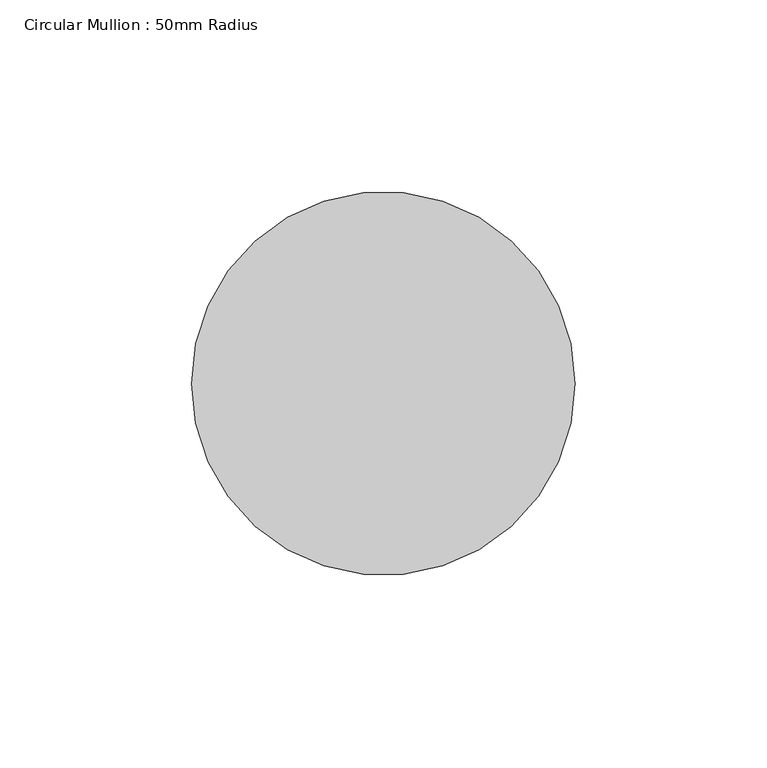
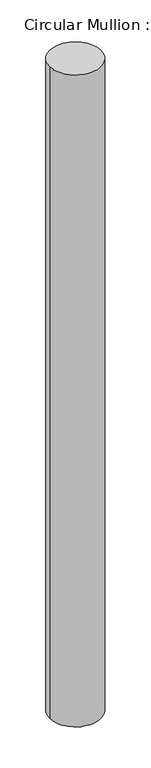
"""IFC4 building model written with IfcOpenShell, lengths in millimetres: member geometry, Circular Mullion : 50mm Radius."""

import ifcopenshell
import ifcopenshell.guid

model = None  # the IFC model being written
_history = None  # IfcOwnerHistory: only IFC2X3 demands one
_inside = {}  # id of a spatial element -> (the spatial element, [elements in it])
_under = {}  # id of a project, library or spatial element -> (it, [spatial elements below it])
_declared = {}  # id of a project -> (the project, [libraries it declares])
_typed = {}  # id of a type object -> (the type object, [elements of that type])
_made_of = {}  # id of a material, layer set ... -> (it, [elements and type objects made of it])


def new_model(schema):
    """Start an empty IFC model of exactly this schema.

    Asked for "IFC4X3", IfcOpenShell would pick the latest addendum, in which some entities
    have other attributes; the version numbers below select the first issue.
    IFC2X3 requires an IfcOwnerHistory on every rooted entity: one is made here for all.
    """
    global model, _history
    if schema == "IFC4X3":
        model = ifcopenshell.file(schema_version=(4, 3, 0, 0))
    else:
        model = ifcopenshell.file(schema=schema)
    _inside.clear()
    _under.clear()
    _declared.clear()
    _typed.clear()
    _made_of.clear()
    _history = None
    if model.schema == "IFC2X3":
        org = make("IfcOrganization", Name="unknown")
        user = make(
            "IfcPersonAndOrganization",
            ThePerson=make("IfcPerson", FamilyName="unknown"),
            TheOrganization=org,
        )
        app = make(
            "IfcApplication",
            ApplicationDeveloper=org,
            Version="unknown",
            ApplicationFullName="unknown",
            ApplicationIdentifier="unknown",
        )
        _history = make(
            "IfcOwnerHistory",
            OwningUser=user,
            OwningApplication=app,
            ChangeAction="ADDED",
            CreationDate=0,
        )
    return model


def make(cls, **values):
    """One entity of the class cls with the attributes given. An attribute that is None is left unset."""
    return model.create_entity(
        cls, **{name: value for name, value in values.items() if value is not None}
    )


def rooted(cls, **values):
    """An entity with a GlobalId (a new one), such as an element, a storey or a relation."""
    return make(cls, GlobalId=ifcopenshell.guid.new(), OwnerHistory=_history, **values)


def si_unit(unit_type, name, prefix=None):
    """IfcSIUnit, for example si_unit("LENGTHUNIT", "METRE", prefix="MILLI")."""
    return make("IfcSIUnit", UnitType=unit_type, Prefix=prefix, Name=name)


def assignment(units):
    """IfcUnitAssignment: the units of a project."""
    return None if units is None else make("IfcUnitAssignment", Units=units)


def point(xyz):
    """IfcCartesianPoint."""
    return None if xyz is None else make("IfcCartesianPoint", Coordinates=xyz)


def direction(xyz):
    """IfcDirection."""
    return None if xyz is None else make("IfcDirection", DirectionRatios=xyz)


def frame(location, z_axis=None, x_axis=None):
    """IfcAxis2Placement3D, a coordinate frame: its origin and axes. An axis left out is left unset."""
    return make(
        "IfcAxis2Placement3D",
        Location=point(location),
        Axis=direction(z_axis),
        RefDirection=direction(x_axis),
    )


def origin():
    """The frame at (0, 0, 0) with its axes left unset."""
    return frame((0.0, 0.0, 0.0))


def place(relative_to, where):
    """IfcLocalPlacement: puts the frame where relative to a parent placement (None: the world)."""
    return make(
        "IfcLocalPlacement", PlacementRelTo=relative_to, RelativePlacement=where
    )


def context(
    kind, dimensions, precision=None, world=None, true_north=None, identifier=None
):
    """IfcGeometricRepresentationContext, for example the 3D "Model" context."""
    return make(
        "IfcGeometricRepresentationContext",
        ContextIdentifier=identifier,
        ContextType=kind,
        CoordinateSpaceDimension=dimensions,
        Precision=precision,
        WorldCoordinateSystem=world,
        TrueNorth=true_north,
    )


def project(units=None, contexts=None):
    """IfcProject with its units and contexts."""
    return rooted(
        "IfcProject",
        Name="project",
        RepresentationContexts=contexts,
        UnitsInContext=assignment(units),
    )


def spatial(cls, under=None, at=None, **own):
    """A site, building, storey or space (cls), placed at a placement, below another one or the project."""
    s = rooted(cls, ObjectPlacement=at, **own)
    if under is not None:
        _under.setdefault(under.id(), (under, []))[1].append(s)
    return s


def ellipse_curve(where, semi_axis1, semi_axis2):
    """IfcEllipse in the frame where."""
    return make(
        "IfcEllipse", Position=where, SemiAxis1=semi_axis1, SemiAxis2=semi_axis2
    )


def shape(context_of_items, identifier, shape_type, items):
    """IfcShapeRepresentation: the items that make up one representation, for example the "Body"."""
    return make(
        "IfcShapeRepresentation",
        ContextOfItems=context_of_items,
        RepresentationIdentifier=identifier,
        RepresentationType=shape_type,
        Items=items,
    )


def source(mapping_origin, context_of_items, identifier, shape_type, items):
    """IfcRepresentationMap: a shape defined once, which mapped items show again and again."""
    return make(
        "IfcRepresentationMap",
        MappingOrigin=mapping_origin,
        MappedRepresentation=shape(context_of_items, identifier, shape_type, items),
    )


def transform(
    local_origin,
    x_axis=None,
    y_axis=None,
    z_axis=None,
    scale=None,
    scale2=None,
    scale3=None,
    uniform=True,
):
    """IfcCartesianTransformationOperator3D, or its non-uniform kind. x_axis, y_axis, z_axis: its Axis1, 2, 3."""
    if uniform:
        return make(
            "IfcCartesianTransformationOperator3D",
            Axis1=direction(x_axis),
            Axis2=direction(y_axis),
            LocalOrigin=point(local_origin),
            Scale=scale,
            Axis3=direction(z_axis),
        )
    return make(
        "IfcCartesianTransformationOperator3DnonUniform",
        Axis1=direction(x_axis),
        Axis2=direction(y_axis),
        LocalOrigin=point(local_origin),
        Scale=scale,
        Axis3=direction(z_axis),
        Scale2=scale2,
        Scale3=scale3,
    )


def mapped(mapping_source, mapping_target):
    """IfcMappedItem: shows the shape of a source again, moved by a transform."""
    return make(
        "IfcMappedItem", MappingSource=mapping_source, MappingTarget=mapping_target
    )


def made_of(thing, what):
    """Note that an element or type object is made of a material, layer set ...; save() writes the relation."""
    if what is not None:
        _made_of.setdefault(what.id(), (what, []))[1].append(thing)
    return thing


def element(
    cls,
    number,
    at=None,
    inside=None,
    cuts=None,
    type_object=None,
    material=None,
    context=None,
    identifier="Body",
    shape_type=None,
    held_by="IfcProductDefinitionShape",
    body=None,
    shapes=None,
    **own,
):
    """One element of the class cls, such as IfcWall. Its Tag is "e" and its number.

    at: its placement. inside: the storey or other place that contains it. cuts: it is an
    opening in that element (IfcRelVoidsElement). A single representation is given by context,
    identifier, shape_type and body (its items); several are given by shapes. held_by: the class
    of the entity that holds the representations. save() writes the other relations.
    """
    e = rooted(cls, Tag="e%d" % number, ObjectPlacement=at, **own)
    if body is not None:
        shapes = [shape(context, identifier, shape_type, body)]
    if shapes is not None:
        e.Representation = make(held_by, Representations=shapes)
    if inside is not None:
        _inside.setdefault(inside.id(), (inside, []))[1].append(e)
    if cuts is not None:
        rooted(
            "IfcRelVoidsElement", RelatingBuildingElement=cuts, RelatedOpeningElement=e
        )
    if type_object is not None:
        _typed.setdefault(type_object.id(), (type_object, []))[1].append(e)
    return made_of(e, material)


def aggregate(whole, parts):
    """IfcRelAggregates: a whole, such as a stair, and the parts it consists of."""
    return rooted("IfcRelAggregates", RelatingObject=whole, RelatedObjects=parts)


def save(model, path):
    """Write the relations noted so far, then the file.

    IfcRelAggregates (storeys below a building ...), IfcRelContainedInSpatialStructure (elements
    in a storey), IfcRelDefinesByType, IfcRelAssociatesMaterial and IfcRelDeclares: one each for
    every whole, place, type object, material and project.
    """
    for whole, parts in _under.values():
        aggregate(whole, parts)
    for where, things in _inside.values():
        rooted(
            "IfcRelContainedInSpatialStructure",
            RelatedElements=things,
            RelatingStructure=where,
        )
    for kind, things in _typed.values():
        rooted("IfcRelDefinesByType", RelatedObjects=things, RelatingType=kind)
    for what, things in _made_of.values():
        rooted("IfcRelAssociatesMaterial", RelatedObjects=things, RelatingMaterial=what)
    for by, libraries in _declared.values():
        rooted("IfcRelDeclares", RelatingContext=by, RelatedDefinitions=libraries)
    model.write(path)


def plane_surface(at):
    """IfcPlane: the flat surface through the origin of the frame at, square to its z axis."""
    return make("IfcPlane", Position=at)


def cylinder_surface(at, radius):
    """IfcCylindricalSurface: all points at the distance radius from the z axis of the frame at."""
    return make("IfcCylindricalSurface", Position=at, Radius=radius)


def advanced_brep(points, edges, surfaces, faces):
    """IfcAdvancedBrep: a solid bounded by faces that lie on surfaces and meet in shared edges.

    An edge is (start, end): straight between two places in points (the first is 0);
    or (start, end, curve); or (start, end, curve, False) where it runs against its curve.
    A face is (place in surfaces, loops), or (place, loops, False) where it looks against
    its surface's normal. A loop lists edges by number (the first is 1), with a minus sign
    where the edge is run from its end to its start. The first loop is the outer one.
    """
    corners = [point(p) for p in points]
    vertices = [make("IfcVertexPoint", VertexGeometry=c) for c in corners]
    made = []
    for start, end, *more in edges:
        made.append(
            make(
                "IfcEdgeCurve",
                EdgeStart=vertices[start],
                EdgeEnd=vertices[end],
                EdgeGeometry=more[0] if more else make("IfcPolyline", Points=[corners[start], corners[end]]),
                SameSense=more[1] if len(more) > 1 else True,
            )
        )
    hull = []
    for where, loops, *sense in faces:
        bounds = []
        for j, loop in enumerate(loops):
            ring = [make("IfcOrientedEdge", EdgeElement=made[abs(k) - 1], Orientation=k > 0) for k in loop]
            bounds.append(
                make(
                    "IfcFaceOuterBound" if j == 0 else "IfcFaceBound",
                    Bound=make("IfcEdgeLoop", EdgeList=ring),
                    Orientation=True,
                )
            )
        hull.append(make("IfcAdvancedFace", Bounds=bounds, FaceSurface=surfaces[where], SameSense=sense[0] if sense else True))
    return make("IfcAdvancedBrep", Outer=make("IfcClosedShell", CfsFaces=hull))


def circular_mullion_50mm_radius_5c607cdf(model_context):
    return source(origin(), model_context, "Body", "AdvancedBrep", [
        advanced_brep(
        [(-100.0, 0.0, 0.8479988), (0.0, 0.0, 0.0), (0.0, 0.0, -1342.2039623), (-100.0, 0.0, -1342.9998247)],
        [
            (0, 1, ellipse_curve(frame((-50.0, 0.0, 0.4239994), z_axis=(-0.008478490448867665, -0.0167700211019321, -0.9998234252066458), x_axis=(-0.45110917903369435, -0.8922709174816219, 0.018791445076169706)), 50.0088303, 50.0)),
            (1, 2),
            (2, 3, ellipse_curve(frame((-50.0, 0.0, -1342.6018935), z_axis=(-0.007957385812667285, -0.01573930274492043, 0.9998444650845111), x_axis=(0.45111867199194494, 0.892289694068219, 0.01763648604081873)), 50.007778, 50.0)),
            (3, 0),
            (1, 0, ellipse_curve(frame((-50.0, 0.0, 0.4239994), z_axis=(-0.008478490448867665, -0.0167700211019321, -0.9998234252066458), x_axis=(-0.45110917903369435, -0.8922709174816219, 0.018791445076169706)), 50.0088303, 50.0)),
            (3, 2, ellipse_curve(frame((-50.0, 0.0, -1342.6018935), z_axis=(-0.007957385812667285, -0.01573930274492043, 0.9998444650845111), x_axis=(0.45111867199194494, 0.892289694068219, 0.01763648604081873)), 50.007778, 50.0)),
        ],
        [
            cylinder_surface(frame((-50.0, 0.0, 0.0), z_axis=(0.0, 0.0, 1.0), x_axis=(1.0, 0.0, 0.0)), 50.0),
            plane_surface(frame((-272.0122061, 137.5223608, 0.0), z_axis=(0.008478490448867667, 0.016770021101932105, 0.999823425206646), x_axis=(0.45110917903369546, 0.8922709174816215, -0.018791445076171982))),
            plane_surface(frame((-272.0122061, 137.5223608, -1342.2039623), z_axis=(0.007957385812667287, 0.015739302744920435, -0.9998444650845113), x_axis=(0.45111867199194505, 0.8922896940682192, 0.017636486040816024))),
        ],
        [
            (0, [[1, 2, 3, 4]]),
            (0, [[5, -4, 6, -2]]),
            (1, [[-1, -5]]),
            (2, [[-6, -3]]),
        ],
    ),
    ])


if __name__ == "__main__":
    model = new_model("IFC4")
    model_context = context("Model", 3, world=origin())
    ifc_project = project(units=[si_unit("LENGTHUNIT", "METRE", prefix="MILLI")], contexts=[model_context])
    site = spatial("IfcSite", under=ifc_project)
    building = spatial("IfcBuilding", under=site)
    placement = place(None, origin())
    circular_mullion_50mm_radius_shape = circular_mullion_50mm_radius_5c607cdf(model_context)
    element("IfcMember", 1, ObjectType="Circular Mullion : 50mm Radius", at=placement, inside=building, context=model_context, shape_type="MappedRepresentation", body=[
        mapped(circular_mullion_50mm_radius_shape, transform((0.0, 0.0, 0.0), x_axis=(1.0, 0.0, 0.0), y_axis=(0.0, 1.0, 0.0), z_axis=(0.0, 0.0, 1.0))),
    ])
    save(model, "model.ifc")

# Revit data of these elements
# Type "Circular Mullion : 50mm Radius"
#   built-in parameter 1007350 = 0.164042 (stored number, unit not read)
# Element 1 (IfcMember, "Circular Mullion : 50mm Radius")
#   Materials on its faces: "Aluminium"
# Materials
#   "Aluminium": class "Metal", colour RGB 247 247 247, transparency 0, Description = "Aluminium 6061", Cost = 0
